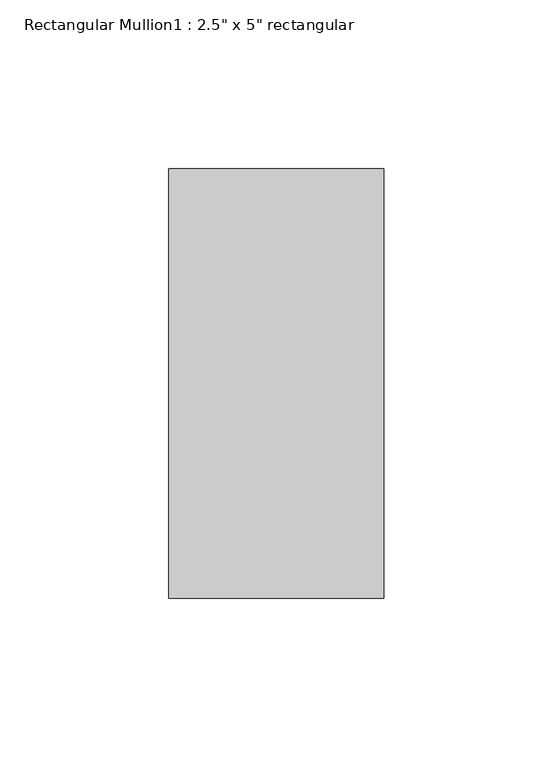
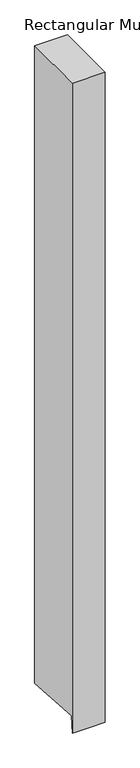
"""IFC4 building model written with IfcOpenShell, lengths in millimetres: member geometry."""

from ifc_helpers import new_model, si_unit, origin, place, context, project, spatial, faceted_brep, source, transform, mapped, element, save


def member_25577aa7(model_context):
    return source(origin(), model_context, "Body", "Brep", [
        faceted_brep([(31.75, 63.5, 0.0), (-31.75, 63.5, 0.0), (-31.75, -63.5, 0.0), (31.75, -63.5, 0.0), (31.75, 63.5, -1307.2809876), (0.0, 63.5, -1307.2809876), (-31.75, 63.5, -1307.2809876), (-31.75, -61.0425175, -1298.2675313), (-31.75, -63.5, -1332.2235469), (0.0, -63.5, -1332.2235469), (31.75, -63.5, -1332.2235469), (31.75, -61.0425175, -1298.2675313), (0.0, -61.0425175, -1298.2675313)], [[[0, 1, 2, 3]], [[1, 0, 4, 5, 6]], [[2, 1, 6, 7, 8]], [[3, 2, 8, 9, 10]], [[0, 3, 10, 11, 4]], [[4, 11, 12, 5]], [[11, 10, 9, 12]], [[9, 8, 7, 12]], [[7, 6, 5, 12]]]),
    ])


if __name__ == "__main__":
    model = new_model("IFC4")
    model_context = context("Model", 3, world=origin())
    ifc_project = project(units=[si_unit("LENGTHUNIT", "METRE", prefix="MILLI")], contexts=[model_context])
    site = spatial("IfcSite", under=ifc_project)
    building = spatial("IfcBuilding", under=site)
    placement = place(None, origin())
    member_shape = member_25577aa7(model_context)
    element("IfcMember", 1, ObjectType="Rectangular Mullion1 : 2.5\" x 5\" rectangular", at=placement, inside=building, context=model_context, shape_type="MappedRepresentation", body=[
        mapped(member_shape, transform((0.0, 0.0, 0.0), x_axis=(1.0, 0.0, 0.0), y_axis=(0.0, 1.0, 0.0), z_axis=(0.0, 0.0, 1.0))),
    ])
    save(model, "model.ifc")

# Revit data of these elements
# Type "Rectangular Mullion1 : 2.5\" x 5\" rectangular"
#   built-in parameter 1007304 = 0.416667 (stored number, unit not read)
#   built-in parameter 1007301 = 0.104167 (stored number, unit not read)
#   built-in parameter 1007300 = 0.104167 (stored number, unit not read)
# Element 1 (IfcMember, "Rectangular Mullion1 : 2.5\" x 5\" rectangular")
#   Materials on its faces: "support-frame"
# Materials
#   "support-frame": class "Unassigned", colour RGB 233 233 233, transparency 0, Cost = 0
